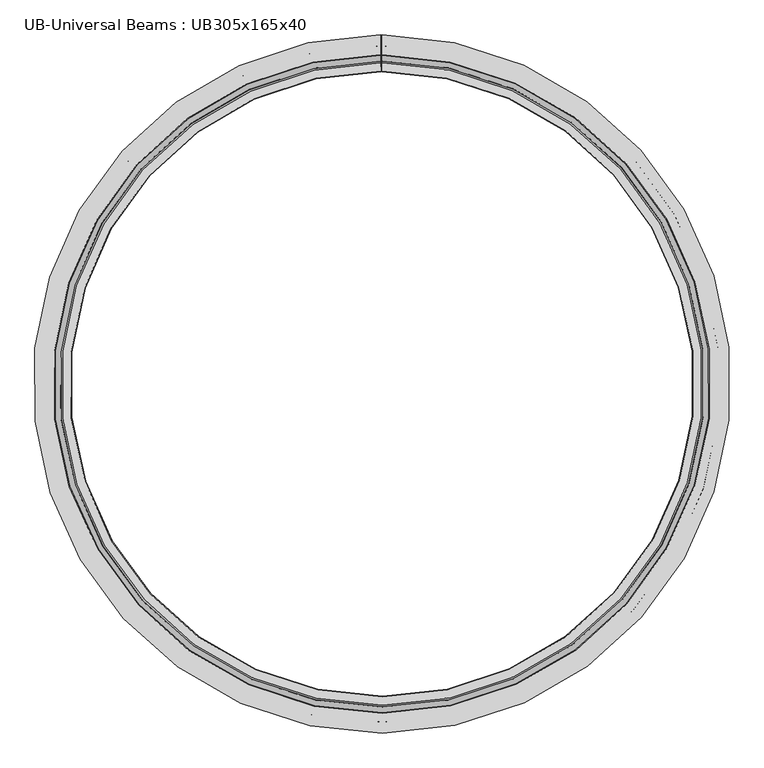
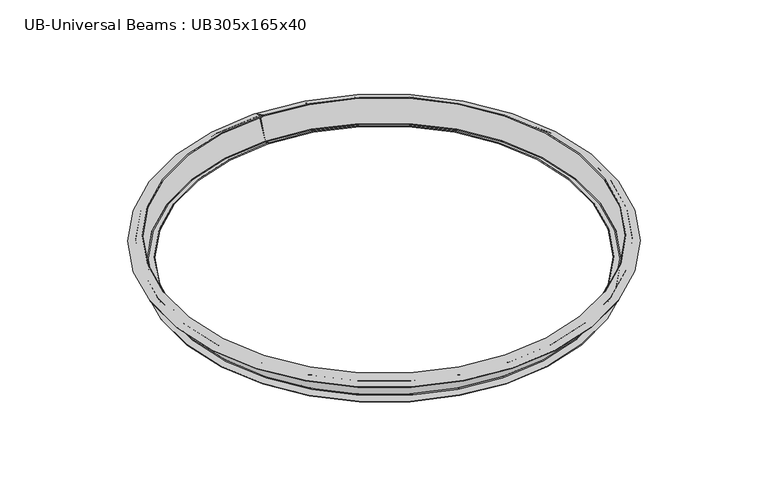
"""IFC4 building model written with IfcOpenShell, lengths in millimetres: beam geometry, UB-Universal Beams : UB305x165x40."""

from ifc_helpers import new_model, si_unit, point, frame, origin, place, context, project, spatial, polyline, circle_curve, ellipse_curve, trimmed, source, transform, mapped, element, save
from ifc_brep_helpers import plane_surface, revolved_surface, advanced_brep


def ub_universal_beams_ub305x165x40_b211cafa(model_context):
    return source(origin(), model_context, "Body", "AdvancedBrep", [
        advanced_brep(
        [(-9.2813175, 14.9526552, -163.1085585), (-9.0434318, -49.0322323, -133.2717092), (-9.0274272, -53.3370394, -121.4442673), (-9.444114, 58.7405491, 118.9085578), (-9.4880863, 70.5679092, 123.2133946), (-9.725972, 134.5527967, 93.3765453), (-9.7419984, 138.8634732, 102.6208847), (-9.1860332, -10.6762782, 172.3528979), (-9.1700068, -14.9869547, 163.1085585), (-9.4078925, 48.9979329, 133.2717092), (-9.4238971, 53.3027399, 121.4442673), (-9.0072103, -58.7748485, -118.9085578), (-8.9632381, -70.6022086, -123.2133946), (-8.7253523, -134.5870962, -93.3765453), (-8.7093259, -138.8977726, -102.6208847), (-9.2652911, 10.6419787, -172.3528979), (0.0, 14.9699084, -163.1085585), (0.0, 10.6592021, -172.3528979), (0.0, -138.8815827, -102.6208847), (0.0, -134.5708765, -93.3765453), (0.0, -70.5855467, -123.2133946), (0.0, -58.7581049, -118.9085578), (0.0, 53.3202581, 121.4442673), (0.0, 49.0154214, 133.2717092), (0.0, -14.9699084, 163.1085585), (0.0, -10.6592021, 172.3528979), (0.0, 138.8815827, 102.6208847), (0.0, 134.5708765, 93.3765453), (0.0, 70.5855467, 123.2133946), (0.0, 58.7581049, 118.9085578), (0.0, -53.3202581, -121.4442673), (0.0, -49.0154214, -133.2717092)],
        [
            (0, 1),
            (1, 2, circle_curve(frame((-9.0574157, -45.2709558, -125.2055699), z_axis=(-0.9999930888962334, -0.0037178165326446095, 0.0), x_axis=(0.0033694860743094072, -0.9063015234494892, 0.4226182617406991)), 8.9)),
            (2, 3),
            (3, 4, circle_curve(frame((-9.4741024, 66.8066326, 115.1472552), z_axis=(-0.9999930888962334, -0.0037178165326453875, 0.0), x_axis=(0.003369486074310112, -0.9063015234494892, 0.42261826174069916)), 8.9)),
            (4, 5),
            (5, 6),
            (6, 7),
            (7, 8),
            (8, 9),
            (9, 10, circle_curve(frame((-9.3939087, 45.2366564, 125.2055699), z_axis=(-0.9999930888962334, -0.0037178165326453875, 0.0), x_axis=(0.003369486074310112, -0.9063015234494892, 0.42261826174069916)), 8.9)),
            (10, 11),
            (11, 12, circle_curve(frame((-8.9772219, -66.8409321, -115.1472552), z_axis=(-0.9999930888962334, -0.0037178165326446095, 0.0), x_axis=(0.0033694860743094072, -0.9063015234494892, 0.4226182617406991)), 8.9)),
            (12, 13),
            (13, 14),
            (14, 15),
            (15, 0),
            (16, 17),
            (17, 18),
            (18, 19),
            (19, 20),
            (20, 21, circle_curve(frame((0.0, -66.8242442, -115.1472552), z_axis=(1.0000000000000002, 0.0, 0.0), x_axis=(0.0, -0.9063077870366502, 0.4226182617406991)), 8.9)),
            (21, 22),
            (22, 23, circle_curve(frame((0.0, 45.2541188, 125.2055699), z_axis=(1.0000000000000002, 0.0, 0.0), x_axis=(0.0, -0.9063077870366502, 0.42261826174069916)), 8.9)),
            (23, 24),
            (24, 25),
            (25, 26),
            (26, 27),
            (27, 28),
            (28, 29, circle_curve(frame((0.0, 66.8242442, 115.1472552), z_axis=(1.0000000000000002, 0.0, 0.0), x_axis=(0.0, -0.9063077870366502, 0.42261826174069916)), 8.9)),
            (29, 30),
            (30, 31, circle_curve(frame((0.0, -45.2541188, -125.2055699), z_axis=(1.0000000000000002, 0.0, 0.0), x_axis=(0.0, -0.9063077870366502, 0.4226182617406991)), 8.9)),
            (31, 16),
            (0, 16, circle_curve(frame((0.0, -2481.473222, -163.1085585), z_axis=(0.0, 0.0, 1.0), x_axis=(-0.9999930888962332, -0.0037178165326318038, 0.0)), 2496.4431304)),
            (31, 1, circle_curve(frame((0.0, -2481.473222, -133.2717092), z_axis=(0.0, 0.0, -1.0), x_axis=(-0.9999930888962332, -0.0037178165326318038, 0.0)), 2432.4578006)),
            (30, 2, circle_curve(frame((0.0, -2481.473222, -121.4442673), z_axis=(0.0, 0.0, -1.0), x_axis=(-0.9999930888962332, -0.0037178165326318038, 0.0)), 2428.1529638)),
            (29, 3, circle_curve(frame((0.0, -2481.473222, 118.9085578), z_axis=(0.0, 0.0, -1.0), x_axis=(-0.9999930888962332, -0.0037178165326318038, 0.0)), 2540.2313268)),
            (28, 4, circle_curve(frame((0.0, -2481.473222, 123.2133946), z_axis=(0.0, 0.0, -1.0), x_axis=(-0.9999930888962332, -0.0037178165326318038, 0.0)), 2552.0587687)),
            (27, 5, circle_curve(frame((0.0, -2481.473222, 93.3765453), z_axis=(0.0, 0.0, -1.0), x_axis=(-0.9999930888962332, -0.0037178165326318038, 0.0)), 2616.0440984)),
            (26, 6, circle_curve(frame((0.0, -2481.473222, 102.6208847), z_axis=(0.0, 0.0, -1.0), x_axis=(-0.9999930888962332, -0.0037178165326318038, 0.0)), 2620.3548047)),
            (25, 7, circle_curve(frame((0.0, -2481.473222, 172.3528979), z_axis=(0.0, 0.0, -1.0), x_axis=(-0.9999930888962332, -0.0037178165326318038, 0.0)), 2470.8140198)),
            (24, 8, circle_curve(frame((0.0, -2481.473222, 163.1085585), z_axis=(0.0, 0.0, -1.0), x_axis=(-0.9999930888962332, -0.0037178165326318038, 0.0)), 2466.5033136)),
            (23, 9, circle_curve(frame((0.0, -2481.473222, 133.2717092), z_axis=(0.0, 0.0, -1.0), x_axis=(-0.9999930888962332, -0.0037178165326318038, 0.0)), 2530.4886433)),
            (22, 10, circle_curve(frame((0.0, -2481.473222, 121.4442673), z_axis=(0.0, 0.0, -1.0), x_axis=(-0.9999930888962332, -0.0037178165326318038, 0.0)), 2534.7934801)),
            (21, 11, circle_curve(frame((0.0, -2481.473222, -118.9085578), z_axis=(0.0, 0.0, -1.0), x_axis=(-0.9999930888962332, -0.0037178165326318038, 0.0)), 2422.7151171)),
            (20, 12, circle_curve(frame((0.0, -2481.473222, -123.2133946), z_axis=(0.0, 0.0, -1.0), x_axis=(-0.9999930888962332, -0.0037178165326318038, 0.0)), 2410.8876753)),
            (19, 13, circle_curve(frame((0.0, -2481.473222, -93.3765453), z_axis=(0.0, 0.0, -1.0), x_axis=(-0.9999930888962332, -0.0037178165326318038, 0.0)), 2346.9023455)),
            (18, 14, circle_curve(frame((0.0, -2481.473222, -102.6208847), z_axis=(0.0, 0.0, -1.0), x_axis=(-0.9999930888962332, -0.0037178165326318038, 0.0)), 2342.5916392)),
            (17, 15, circle_curve(frame((0.0, -2481.473222, -172.3528979), z_axis=(0.0, 0.0, -1.0), x_axis=(-0.9999930888962332, -0.0037178165326318038, 0.0)), 2492.1324241)),
        ],
        [
            plane_surface(frame((-9.2256622, -0.0171497, 0.0), z_axis=(0.9999930888962332, 0.0037178165326321104, 0.0), x_axis=(-0.0015712171604918153, 0.42261534098203835, 0.9063077870366502))),
            plane_surface(frame((0.0, 0.0, 0.0), z_axis=(-1.0, 0.0, 0.0), x_axis=(0.0, 0.422618261740699, 0.9063077870366502))),
            revolved_surface(polyline([(-2432.4409896, -2490.5166538, -133.2717092), (-2496.4258772, -2490.7545395, -163.1085585)]), (0.0, -2481.473222, 0.0), (0.0, 0.0, -1.0)),
            revolved_surface(trimmed(ellipse_curve(frame((-2436.2022662, -2490.5306376, -125.2055699), z_axis=(-0.0037178165326371983, 0.9999930888962334, 0.0), x_axis=(0.9063015234494892, 0.00336948607430269, 0.4226182617406992)), 8.9, 8.9), [point((-2428.1361826, -2490.5006492, -121.4442673))], [point((-2432.4409896, -2490.5166538, -133.2717092))], True, "CARTESIAN"), (0.0, -2481.473222, 0.0), (0.0, 0.0, -1.0)),
            revolved_surface(polyline([(-2540.213771, -2490.917336, 118.9085578), (-2428.1361826, -2490.5006492, -121.4442673)]), (0.0, -2481.473222, 0.0), (0.0, 0.0, -1.0)),
            revolved_surface(trimmed(ellipse_curve(frame((-2548.2798546, -2490.9473244, 115.1472552), z_axis=(-0.003717816532637976, 0.9999930888962334, 0.0), x_axis=(0.9063015234494892, 0.0033694860743033947, 0.4226182617406993)), 8.9, 8.9), [point((-2552.0411311, -2490.9613082, 123.2133946))], [point((-2540.213771, -2490.917336, 118.9085578))], True, "CARTESIAN"), (0.0, -2481.473222, 0.0), (0.0, 0.0, -1.0)),
            revolved_surface(polyline([(-2616.0260187, -2491.199194, 93.3765453), (-2552.0411311, -2490.9613082, 123.2133946)]), (0.0, -2481.473222, 0.0), (0.0, 0.0, -1.0)),
            revolved_surface(polyline([(-2620.3366952, -2491.2152204, 102.6208847), (-2616.0260187, -2491.199194, 93.3765453)]), (0.0, -2481.473222, 0.0), (0.0, 0.0, -1.0)),
            revolved_surface(polyline([(-2470.7969438, -2490.6592552, 172.3528979), (-2620.3366952, -2491.2152204, 102.6208847)]), (0.0, -2481.473222, 0.0), (0.0, 0.0, -1.0)),
            revolved_surface(polyline([(-2466.4862673, -2490.6432288, 163.1085585), (-2470.7969438, -2490.6592552, 172.3528979)]), (0.0, -2481.473222, 0.0), (0.0, 0.0, -1.0)),
            revolved_surface(polyline([(-2530.4711549, -2490.8811145, 133.2717092), (-2466.4862673, -2490.6432288, 163.1085585)]), (0.0, -2481.473222, 0.0), (0.0, 0.0, -1.0)),
            revolved_surface(trimmed(ellipse_curve(frame((-2526.7098783, -2490.8671306, 125.2055699), z_axis=(-0.003717816532637976, 0.9999930888962334, 0.0), x_axis=(0.9063015234494892, 0.0033694860743033947, 0.4226182617406993)), 8.9, 8.9), [point((-2534.7759619, -2490.8971191, 121.4442673))], [point((-2530.4711549, -2490.8811145, 133.2717092))], True, "CARTESIAN"), (0.0, -2481.473222, 0.0), (0.0, 0.0, -1.0)),
            revolved_surface(polyline([(-2422.6983735, -2490.4804323, -118.9085578), (-2534.7759619, -2490.8971191, 121.4442673)]), (0.0, -2481.473222, 0.0), (0.0, 0.0, -1.0)),
            revolved_surface(trimmed(ellipse_curve(frame((-2414.6322899, -2490.4504439, -115.1472552), z_axis=(-0.0037178165326371983, 0.9999930888962334, 0.0), x_axis=(0.9063015234494892, 0.00336948607430269, 0.4226182617406992)), 8.9, 8.9), [point((-2410.8710134, -2490.43646, -123.2133946))], [point((-2422.6983735, -2490.4804323, -118.9085578))], True, "CARTESIAN"), (0.0, -2481.473222, 0.0), (0.0, 0.0, -1.0)),
            revolved_surface(polyline([(-2346.8861258, -2490.1985743, -93.3765453), (-2410.8710134, -2490.43646, -123.2133946)]), (0.0, -2481.473222, 0.0), (0.0, 0.0, -1.0)),
            revolved_surface(polyline([(-2342.5754493, -2490.1825479, -102.6208847), (-2346.8861258, -2490.1985743, -93.3765453)]), (0.0, -2481.473222, 0.0), (0.0, 0.0, -1.0)),
            revolved_surface(polyline([(-2492.1152007, -2490.7385131, -172.3528979), (-2342.5754493, -2490.1825479, -102.6208847)]), (0.0, -2481.473222, 0.0), (0.0, 0.0, -1.0)),
            revolved_surface(polyline([(-2496.4258772, -2490.7545395, -163.1085585), (-2492.1152007, -2490.7385131, -172.3528979)]), (0.0, -2481.473222, 0.0), (0.0, 0.0, -1.0)),
        ],
        [
            (0, [[1, 2, 3, 4, 5, 6, 7, 8, 9, 10, 11, 12, 13, 14, 15, 16]]),
            (1, [[17, 18, 19, 20, 21, 22, 23, 24, 25, 26, 27, 28, 29, 30, 31, 32]]),
            (2, [[-1, 33, -32, 34]]),
            (3, [[-2, -34, -31, 35]]),
            (4, [[-3, -35, -30, 36]]),
            (5, [[-4, -36, -29, 37]]),
            (6, [[-5, -37, -28, 38]]),
            (7, [[-6, -38, -27, 39]]),
            (8, [[-7, -39, -26, 40]]),
            (9, [[-8, -40, -25, 41]]),
            (10, [[-9, -41, -24, 42]]),
            (11, [[-10, -42, -23, 43]]),
            (12, [[-11, -43, -22, 44]]),
            (13, [[-12, -44, -21, 45]]),
            (14, [[-13, -45, -20, 46]]),
            (15, [[-14, -46, -19, 47]]),
            (16, [[-15, -47, -18, 48]]),
            (17, [[-16, -48, -17, -33]]),
        ],
    ),
    ])


if __name__ == "__main__":
    model = new_model("IFC4")
    model_context = context("Model", 3, world=origin())
    ifc_project = project(units=[si_unit("LENGTHUNIT", "METRE", prefix="MILLI")], contexts=[model_context])
    site = spatial("IfcSite", under=ifc_project)
    building = spatial("IfcBuilding", under=site)
    placement = place(None, origin())
    ub_universal_beams_ub305x165x40_shape = ub_universal_beams_ub305x165x40_b211cafa(model_context)
    element("IfcBeam", 1, ObjectType="UB-Universal Beams : UB305x165x40", at=placement, inside=building, context=model_context, shape_type="MappedRepresentation", body=[
        mapped(ub_universal_beams_ub305x165x40_shape, transform((0.0, 0.0, 0.0), x_axis=(1.0, 0.0, 0.0), y_axis=(0.0, 1.0, 0.0), z_axis=(0.0, 0.0, 1.0))),
    ])
    save(model, "model.ifc")

# Revit data of these elements
# Type "UB-Universal Beams : UB305x165x40"
#   Section Name Key = "UB305X165X40"
#   Width = 16.5 cm
#   Web Thickness = 0.6 cm
#   Web Fillet = 0.89 cm
#   Warping Constant = 164000.0 cm⁶
#   Torsional Moment of Inertia = 14.70 cm⁴
#   Section Area = 51.3 cm²
#   Plastic Modulus weak axis = 142.0 cm³
#   Plastic Modulus strong axis = 623.0 cm³
#   Nominal Weight = 40.2999 kgf/m
#   Moment of Inertia weak axis = 764.00 cm⁴
#   Moment of Inertia strong axis = 8503.00 cm⁴
#   Height = 30.34 cm
#   Flange Thickness = 1.02 cm
#   Elastic Modulus weak axis = 92.6 cm³
#   Elastic Modulus strong axis = 560.0 cm³
#   Centroid Vertical = 15.17 cm
#   Centroid Horizontal = 8.25 cm
#   Bolt Spacing = 9.0 cm
#   Length [instance default] = 1500 mm
#   Structural Material [instance default] = Metal - Steel 43-275
#   Type Comments = ""
#   Assembly Code = ""
# Element 1 (IfcBeam, "UB-Universal Beams : UB305x165x40")
#   Materials on its faces: "Metal - Steel 43-275"
# Materials
#   "Metal - Steel 43-275": class "Metal", colour RGB 247 247 247, transparency 0, Cost = 0
